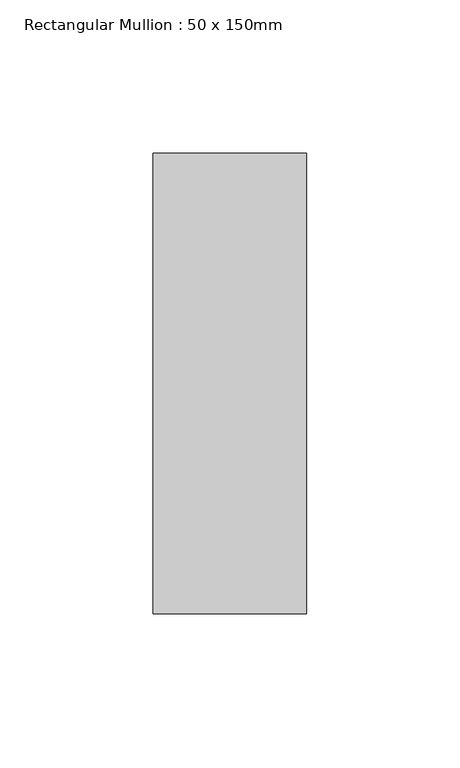
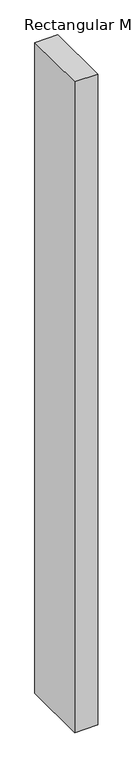
"""IFC4 building model written with IfcOpenShell, lengths in millimetres: member geometry, Rectangular Mullion : 50 x 150mm."""

from ifc_helpers import new_model, si_unit, frame, origin, place, context, project, spatial, polyline, outline, extrude, source, transform, mapped, element, save


def rectangular_mullion_50_x_150mm_964d2677(model_context):
    return source(origin(), model_context, "Body", "SweptSolid", [
        extrude(outline(polyline([(25.0, 75.0), (25.0, -75.0), (-25.0, -75.0), (-25.0, 75.0), (25.0, 75.0)])), frame((0.0, 0.0, -1500.0), z_axis=(0.0, 0.0, 1.0), x_axis=(1.0, 0.0, 0.0)), (0.0, 0.0, 1.0), 1500.0),
    ])


if __name__ == "__main__":
    model = new_model("IFC4")
    model_context = context("Model", 3, world=origin())
    ifc_project = project(units=[si_unit("LENGTHUNIT", "METRE", prefix="MILLI")], contexts=[model_context])
    site = spatial("IfcSite", under=ifc_project)
    building = spatial("IfcBuilding", under=site)
    placement = place(None, origin())
    rectangular_mullion_50_x_150mm_shape = rectangular_mullion_50_x_150mm_964d2677(model_context)
    element("IfcMember", 1, ObjectType="Rectangular Mullion : 50 x 150mm", at=placement, inside=building, context=model_context, shape_type="MappedRepresentation", body=[
        mapped(rectangular_mullion_50_x_150mm_shape, transform((0.0, 0.0, 0.0), x_axis=(1.0, 0.0, 0.0), y_axis=(0.0, 1.0, 0.0), z_axis=(0.0, 0.0, 1.0))),
    ])
    save(model, "model.ifc")

# Revit data of these elements
# Type "Rectangular Mullion : 50 x 150mm"
#   built-in parameter 1007304 = 0.492126 (stored number, unit not read)
#   built-in parameter 1007301 = 0.082021 (stored number, unit not read)
#   built-in parameter 1007300 = 0.082021 (stored number, unit not read)
# Element 1 (IfcMember, "Rectangular Mullion : 50 x 150mm")
#   Materials on its faces: "Metal - Aluminium"
# Materials
#   "Metal - Aluminium": class "Metal", colour RGB 247 247 247, transparency 0
